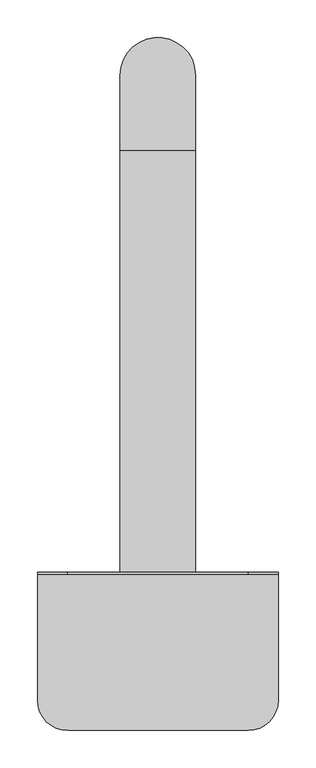
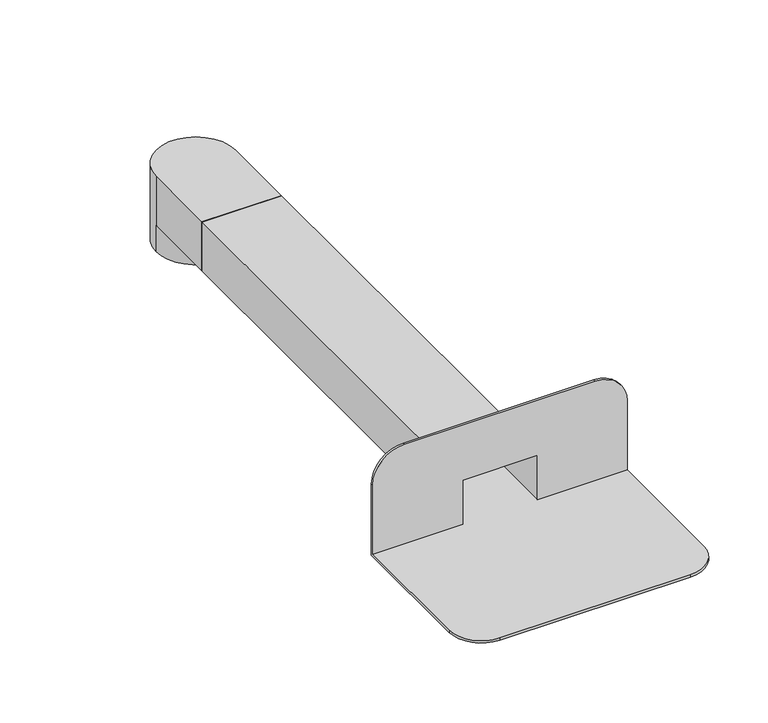
"""IFC4 building model written with IfcOpenShell, lengths in millimetres: proxy geometry, TN_ПВХ воронка парапетная : ПВХ воронка парапетная 65х100мм длиной 550мм с отводом Ø100мм."""

from ifc_helpers import new_model, si_unit, frame, origin, place, context, project, spatial, polyline, circle_curve, source, transform, mapped, element, save
from ifc_brep_helpers import plane_surface, cylinder_surface, revolved_surface, advanced_brep


def specialty_equipment_5b4f2acb(model_context):
    return source(origin(), model_context, "Body", "AdvancedBrep", [
        advanced_brep(
        [(-50.0, 660.0, -35.0), (50.0, 660.0, -35.0), (-47.0, 660.0, -35.0), (47.0, 660.0, -35.0), (-47.0, 642.9412779, 3.0), (47.0, 642.9412779, 3.0), (47.0, 642.9412779, 62.0), (-47.0, 642.9412779, 62.0), (50.0, 660.0, 0.0), (-50.0, 660.0, 0.0), (-50.0, 660.0, 65.0), (50.0, 660.0, 65.0), (-47.0, 660.0, 62.0), (47.0, 660.0, 62.0), (50.0, 560.0, 0.0), (50.0, 560.0, 65.0), (-50.0, 560.0, 65.0), (-50.0, 560.0, 0.0), (47.0, 560.0, 3.0), (-47.0, 560.0, 3.0), (-47.0, 560.0, 62.0), (47.0, 560.0, 62.0)],
        [
            (0, 1, circle_curve(frame((0.0, 660.0, -35.0), z_axis=(0.0, 0.0, -1.0), x_axis=(1.0, 0.0, 0.0)), 50.0)),
            (1, 0, circle_curve(frame((0.0, 660.0, -35.0), z_axis=(0.0, 0.0, -1.0), x_axis=(1.0, 0.0, 0.0)), 50.0)),
            (2, 3, circle_curve(frame((0.0, 660.0, -35.0), z_axis=(0.0, 0.0, 1.0), x_axis=(1.0, 0.0, 0.0)), 47.0)),
            (3, 2, circle_curve(frame((0.0, 660.0, -35.0), z_axis=(0.0, 0.0, 1.0), x_axis=(1.0, 0.0, 0.0)), 47.0)),
            (4, 5, circle_curve(frame((0.0, 660.0, 3.0), z_axis=(0.0, 0.0, 1.0), x_axis=(1.0, 0.0, 0.0)), 50.0)),
            (5, 6),
            (6, 7, circle_curve(frame((0.0, 660.0, 62.0), z_axis=(0.0, 0.0, -1.0), x_axis=(1.0, 0.0, 0.0)), 50.0)),
            (7, 4),
            (1, 8),
            (8, 9, circle_curve(frame((0.0, 660.0, 0.0), z_axis=(0.0, 0.0, -1.0), x_axis=(1.0, 0.0, 0.0)), 50.0)),
            (9, 0),
            (10, 11, circle_curve(frame((0.0, 660.0, 65.0), z_axis=(0.0, 0.0, -1.0), x_axis=(1.0, 0.0, 0.0)), 50.0)),
            (11, 8),
            (9, 10),
            (12, 13, circle_curve(frame((0.0, 660.0, 62.0), z_axis=(0.0, 0.0, -1.0), x_axis=(1.0, 0.0, 0.0)), 47.0)),
            (13, 12, circle_curve(frame((0.0, 660.0, 62.0), z_axis=(0.0, 0.0, -1.0), x_axis=(1.0, 0.0, 0.0)), 47.0)),
            (13, 3),
            (2, 12),
            (14, 15),
            (15, 16),
            (16, 17),
            (17, 14),
            (18, 19),
            (19, 20),
            (20, 21),
            (21, 18),
            (14, 8),
            (11, 15),
            (10, 16),
            (9, 17),
            (18, 5),
            (4, 19),
            (7, 20),
            (6, 21),
        ],
        [
            plane_surface(frame((50.0, 660.0, -35.0), z_axis=(0.0, 0.0, -1.0), x_axis=(0.0, -1.0, 0.0))),
            cylinder_surface(frame((0.0, 660.0, -35.0), z_axis=(0.0, 0.0, 1.0), x_axis=(1.0, 0.0, 0.0)), 50.0),
            plane_surface(frame((47.0, 660.0, 62.0), z_axis=(0.0, 0.0, -1.0), x_axis=(0.0, 1.0, 0.0))),
            revolved_surface(polyline([(47.0, 660.0, 62.0), (47.0, 660.0, -35.0)]), (0.0, 660.0, -35.0), (0.0, 0.0, 1.0)),
            plane_surface(frame((-50.0, 560.0, 0.0), z_axis=(0.0, -1.0, 0.0), x_axis=(1.0, 0.0, 0.0))),
            plane_surface(frame((50.0, 660.0, 65.0), z_axis=(1.0, 0.0, 0.0), x_axis=(0.0, -1.0, 0.0))),
            plane_surface(frame((-50.0, 660.0, 65.0), z_axis=(0.0, 0.0, 1.0), x_axis=(0.0, -1.0, 0.0))),
            plane_surface(frame((-50.0, 660.0, 0.0), z_axis=(-1.0, 0.0, 0.0), x_axis=(0.0, -1.0, 0.0))),
            plane_surface(frame((50.0, 660.0, 0.0), z_axis=(0.0, 0.0, -1.0), x_axis=(0.0, -1.0, 0.0))),
            plane_surface(frame((-47.0, 660.0, 3.0), z_axis=(0.0, 0.0, 1.0), x_axis=(0.0, -1.0, 0.0))),
            plane_surface(frame((-47.0, 660.0, 62.0), z_axis=(1.0, 0.0, 0.0), x_axis=(0.0, -1.0, 0.0))),
            plane_surface(frame((47.0, 660.0, 62.0), z_axis=(0.0, 0.0, -1.0), x_axis=(0.0, -1.0, 0.0))),
            plane_surface(frame((47.0, 660.0, 3.0), z_axis=(-1.0, 0.0, 0.0), x_axis=(0.0, -1.0, 0.0))),
        ],
        [
            (0, [[1, 2], [3, 4]]),
            (1, [[5, 6, 7, 8]]),
            (1, [[-2, 9, 10, 11]]),
            (1, [[12, 13, -9, -1, -11, 14]]),
            (2, [[15, 16]]),
            (3, [[-16, 17, -3, 18]]),
            (3, [[-15, -18, -4, -17]]),
            (4, [[19, 20, 21, 22], [23, 24, 25, 26]]),
            (5, [[-19, 27, -13, 28]]),
            (6, [[-20, -28, -12, 29]]),
            (7, [[-21, -29, -14, 30]]),
            (8, [[-22, -30, -10, -27]]),
            (9, [[-23, 31, -5, 32]]),
            (10, [[-24, -32, -8, 33]]),
            (11, [[-25, -33, -7, 34]]),
            (12, [[-26, -34, -6, -31]]),
        ],
    ),
        advanced_brep(
        [(50.0, 560.0, 0.0), (50.0, 560.0, 65.0), (50.0, 0.0, 65.0), (50.0, 0.0, 0.0), (-50.0, 560.0, 65.0), (-50.0, 0.0, 65.0), (-50.0, 560.0, 0.0), (-50.0, 0.0, 0.0), (160.0, -3.0, 3.0), (160.0, -3.0, 95.0), (120.0, -3.0, 135.0), (-120.0, -3.0, 135.0), (-160.0, -3.0, 95.0), (-160.0, -3.0, 3.0), (-47.0, -3.0, 3.0), (-47.0, -3.0, 62.0), (47.0, -3.0, 62.0), (47.0, -3.0, 3.0), (-160.0, 0.0, 95.0), (-120.0, 0.0, 135.0), (120.0, 0.0, 135.0), (160.0, 0.0, 95.0), (160.0, 0.0, 0.0), (-160.0, 0.0, 0.0), (160.0, -170.0, 3.0), (160.0, -170.0, 0.0), (-160.0, -170.0, 0.0), (-160.0, -170.0, 3.0), (-120.0, -210.0, 3.0), (-120.0, -210.0, 0.0), (120.0, -210.0, 3.0), (120.0, -210.0, 0.0), (47.0, 560.0, 3.0), (47.0, 560.0, 62.0), (-47.0, 560.0, 62.0), (-47.0, 560.0, 3.0)],
        [
            (0, 1),
            (1, 2),
            (2, 3),
            (3, 0),
            (1, 4),
            (4, 5),
            (5, 2),
            (4, 6),
            (6, 7),
            (7, 5),
            (8, 9),
            (9, 10, circle_curve(frame((120.0, -3.0, 95.0), z_axis=(0.0, -1.0, 0.0), x_axis=(1.0, 0.0, 0.0)), 40.0)),
            (10, 11),
            (11, 12, circle_curve(frame((-120.0, -3.0, 95.0), z_axis=(0.0, -1.0, 0.0), x_axis=(1.0, 0.0, 0.0)), 40.0)),
            (12, 13),
            (13, 14),
            (14, 15),
            (15, 16),
            (16, 17),
            (17, 8),
            (18, 19, circle_curve(frame((-120.0, 0.0, 95.0), z_axis=(0.0, 1.0, 0.0), x_axis=(1.0, 0.0, 0.0)), 40.0)),
            (19, 20),
            (20, 21, circle_curve(frame((120.0, 0.0, 95.0), z_axis=(0.0, 1.0, 0.0), x_axis=(1.0, 0.0, 0.0)), 40.0)),
            (21, 22),
            (22, 3),
            (7, 23),
            (23, 18),
            (8, 24),
            (24, 25),
            (25, 22),
            (21, 9),
            (20, 10),
            (19, 11),
            (18, 12),
            (23, 26),
            (26, 27),
            (27, 13),
            (28, 27, circle_curve(frame((-120.0, -170.0, 3.0), z_axis=(0.0, 0.0, -1.0), x_axis=(1.0, 0.0, 0.0)), 40.0)),
            (26, 29, circle_curve(frame((-120.0, -170.0, 0.0), z_axis=(0.0, 0.0, 1.0), x_axis=(1.0, 0.0, 0.0)), 40.0)),
            (29, 28),
            (30, 28),
            (29, 31),
            (31, 30),
            (24, 30, circle_curve(frame((120.0, -170.0, 3.0), z_axis=(0.0, 0.0, -1.0), x_axis=(1.0, 0.0, 0.0)), 40.0)),
            (31, 25, circle_curve(frame((120.0, -170.0, 0.0), z_axis=(0.0, 0.0, 1.0), x_axis=(1.0, 0.0, 0.0)), 40.0)),
            (0, 6),
            (32, 33),
            (33, 34),
            (34, 35),
            (35, 32),
            (35, 14),
            (17, 32),
            (34, 15),
            (33, 16),
        ],
        [
            plane_surface(frame((50.0, 0.0, 0.0), z_axis=(1.0, 0.0, 0.0), x_axis=(0.0, 1.0, 0.0))),
            plane_surface(frame((50.0, 0.0, 65.0), z_axis=(0.0, 0.0, 1.0), x_axis=(0.0, 1.0, 0.0))),
            plane_surface(frame((-50.0, 0.0, 65.0), z_axis=(-1.0, 0.0, 0.0), x_axis=(0.0, 1.0, 0.0))),
            plane_surface(frame((160.0, -3.0, 95.0), z_axis=(0.0, -1.0, 0.0), x_axis=(0.0, 0.0, 1.0))),
            plane_surface(frame((160.0, 0.0, 95.0), z_axis=(0.0, 1.0, 0.0), x_axis=(0.0, 0.0, -1.0))),
            plane_surface(frame((160.0, -3.0, 3.0), z_axis=(1.0, 0.0, 0.0), x_axis=(0.0, 1.0, 0.0))),
            cylinder_surface(frame((120.0, 0.0, 95.0), z_axis=(0.0, -1.0, 0.0), x_axis=(1.0, 0.0, 0.0)), 40.0),
            plane_surface(frame((120.0, -3.0, 135.0), z_axis=(0.0, 0.0, 1.0), x_axis=(0.0, 1.0, 0.0))),
            cylinder_surface(frame((-120.0, 0.0, 95.0), z_axis=(0.0, -1.0, 0.0), x_axis=(1.0, 0.0, 0.0)), 40.0),
            plane_surface(frame((-160.0, -3.0, 95.0), z_axis=(-1.0, 0.0, 0.0), x_axis=(0.0, 1.0, 0.0))),
            cylinder_surface(frame((-120.0, -170.0, 0.0), z_axis=(0.0, 0.0, 1.0), x_axis=(1.0, 0.0, 0.0)), 40.0),
            plane_surface(frame((-120.0, -210.0, 3.0), z_axis=(0.0, -1.0, 0.0), x_axis=(0.0, 0.0, -1.0))),
            cylinder_surface(frame((120.0, -170.0, 0.0), z_axis=(0.0, 0.0, 1.0), x_axis=(1.0, 0.0, 0.0)), 40.0),
            plane_surface(frame((50.0, 560.0, 0.0), z_axis=(0.0, 1.0, 0.0), x_axis=(0.0, 0.0, -1.0))),
            plane_surface(frame((-50.0, 0.0, 0.0), z_axis=(0.0, 0.0, -1.0), x_axis=(0.0, 1.0, 0.0))),
            plane_surface(frame((47.0, 0.0, 3.0), z_axis=(0.0, 0.0, 1.0), x_axis=(0.0, 1.0, 0.0))),
            plane_surface(frame((-47.0, 0.0, 3.0), z_axis=(1.0, 0.0, 0.0), x_axis=(0.0, 1.0, 0.0))),
            plane_surface(frame((-47.0, 0.0, 62.0), z_axis=(0.0, 0.0, -1.0), x_axis=(0.0, 1.0, 0.0))),
            plane_surface(frame((47.0, 0.0, 62.0), z_axis=(-1.0, 0.0, 0.0), x_axis=(0.0, 1.0, 0.0))),
        ],
        [
            (0, [[1, 2, 3, 4]]),
            (1, [[5, 6, 7, -2]]),
            (2, [[8, 9, 10, -6]]),
            (3, [[11, 12, 13, 14, 15, 16, 17, 18, 19, 20]]),
            (4, [[21, 22, 23, 24, 25, -3, -7, -10, 26, 27]]),
            (5, [[-11, 28, 29, 30, -24, 31]]),
            (6, [[-12, -31, -23, 32]]),
            (7, [[-13, -32, -22, 33]]),
            (8, [[-14, -33, -21, 34]]),
            (9, [[-15, -34, -27, 35, 36, 37]]),
            (10, [[38, -36, 39, 40]]),
            (11, [[41, -40, 42, 43]]),
            (12, [[44, -43, 45, -29]]),
            (13, [[46, -8, -5, -1], [47, 48, 49, 50]]),
            (14, [[-46, -4, -25, -30, -45, -42, -39, -35, -26, -9]]),
            (15, [[-50, 51, -16, -37, -38, -41, -44, -28, -20, 52]]),
            (16, [[-51, -49, 53, -17]]),
            (17, [[-48, 54, -18, -53]]),
            (18, [[-47, -52, -19, -54]]),
        ],
    ),
    ])


if __name__ == "__main__":
    model = new_model("IFC4")
    model_context = context("Model", 3, world=origin())
    ifc_project = project(units=[si_unit("LENGTHUNIT", "METRE", prefix="MILLI")], contexts=[model_context])
    site = spatial("IfcSite", under=ifc_project)
    building = spatial("IfcBuilding", under=site)
    placement = place(None, origin())
    specialty_equipment_shape = specialty_equipment_5b4f2acb(model_context)
    element("IfcBuildingElementProxy", 1, Name="TN_ПВХ воронка парапетная : ПВХ воронка парапетная 65х100мм длиной 550мм с отводом Ø100мм", ObjectType="TN_ПВХ воронка парапетная : ПВХ воронка парапетная 65х100мм длиной 550мм с отводом Ø100мм", at=placement, inside=building, context=model_context, shape_type="MappedRepresentation", body=[
        mapped(specialty_equipment_shape, transform((0.0, 0.0, 0.0), x_axis=(1.0, 0.0, 0.0), y_axis=(0.0, 1.0, 0.0), z_axis=(0.0, 0.0, 1.0))),
    ])
    save(model, "model.ifc")

# Revit data of these elements
# Type "TN_ПВХ воронка парапетная : ПВХ воронка парапетная 65х100мм длиной 550мм с отводом Ø100мм"
#   ADSK_Группирование = "Комплектующие и воронки"
#   Description = "ПВХ воронка парапетная ТехноНИКОЛЬ – кровельная воронка для отвода воды через балконы и парапеты на плоской кровле. Воронка имеет квадратное сечение отводящей трубы. Применяется совместно с ПВХ мембранами LOGICROOF и ECOPLAST. Приваривается к мембране гомогенно при помощи горячего воздуха. В состав комплекта входит Корпус воронки из ПВХ, угловой отвод из полипропилена и элемент жёсткости из алюминия. Угловой отвод воронки предназначен для соединения с водосточными трубами диаметром 100 мм. Масса 930 г. Пропускная способность не менее 8 л/с."
#   Manufacturer = "ТехноНИКОЛЬ"
#   URL = "http://nav.tn.ru/catalog/krovlya/komplektatsiya/pvkh-aerator-krovelnyy-tekhnonikol/"
#   ADSK_Примечание = ""
#   ADSK_Обозначение = "ТехноНИКОЛЬ"
#   ADSK_Наименование = "ПВХ воронка парапетная 65х100мм длиной 550мм с отводом Ø100мм"
#   ADSK_Марка = ""
#   ADSK_Код изделия = "571218"
#   ADSK_Завод-изготовитель = "ТехноНИКОЛЬ"
#   ADSK_Единица измерения = "шт."
#   ADSK_Группирование = "Комплектующие и воронки"
#   ADSK_URL страницы изделия = "https://shop.tn.ru/pvh-voronka-parapetnaja-65h100-mm-dlinoj-550-mm-s-otvodom-o100-mm"
#   ADSK_URL документации изделия = "https://nav.tn.ru/upload/iblock/003/Tekhlist-7.64_Parapetnaya-voronka_rus.pdf"
#   Тип воронки = 1
#   Длина расчетная [instance default] = 560 mm
#   Длина отвода [instance default] = 560 mm
#   ADSK_Размер_Ширина = 100 mm
#   ADSK_Размер_Высота = 65 mm
#   ADSK_Количество = 1
#   Видимость_Переход [instance default] = yes
#   Видимость_Листоуловитель [instance default] = no
#   Видимость отвода [instance default] = yes
#   Видимость листоуловителя [instance default] = no
#   Материал_Листоуловитель = TN_ПВХ_Черный
#   Материал_Корпус = TN_ПВХ_Серый
#   Default Elevation = 0
# Element 1 (IfcBuildingElementProxy, "TN_ПВХ воронка парапетная : ПВХ воронка парапетная 65х100мм длиной 550мм с отводом Ø100мм")
#   Materials on its faces: "TN_ПВХ_Серый"
# Materials
#   "TN_ПВХ_Черный": class "Типовые", colour RGB 48 48 48, transparency 0, Cost = 0
#   "TN_ПВХ_Серый": class "Типовые", colour RGB 192 192 192, transparency 0, Cost = 0
